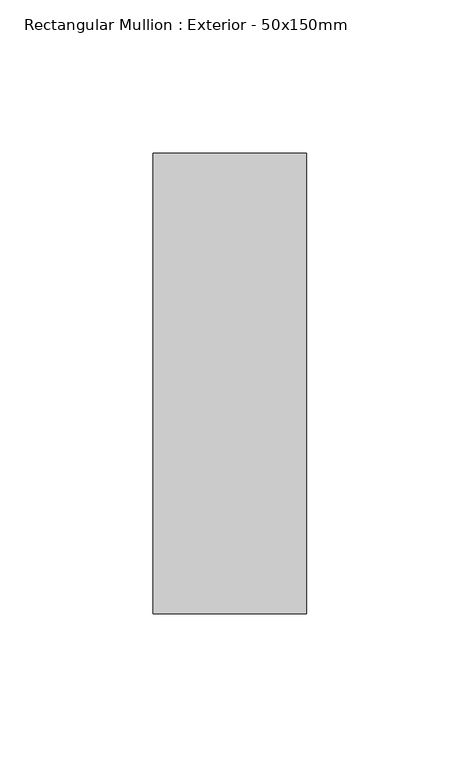
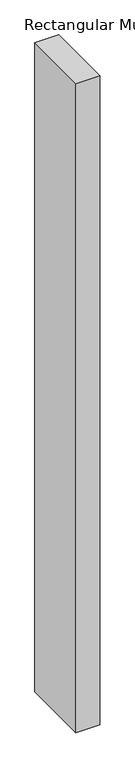
"""IFC4 building model written with IfcOpenShell, lengths in millimetres: member geometry, Rectangular Mullion : Exterior - 50x150mm."""

from ifc_helpers import new_model, si_unit, frame, origin, place, context, project, spatial, polyline, outline, extrude, source, transform, mapped, element, save


def rectangular_mullion_exterior_50x150mm_c96db089(model_context):
    return source(origin(), model_context, "Body", "SweptSolid", [
        extrude(outline(polyline([(0.0, 0.0), (0.0, -150.0), (-50.0, -150.0), (-50.0, 0.0), (0.0, 0.0)])), frame((0.0, 0.0, -1449.9999999), z_axis=(0.0, 0.0, 1.0), x_axis=(1.0, 0.0, 0.0)), (0.0, 0.0, 1.0), 1449.9999999),
    ])


if __name__ == "__main__":
    model = new_model("IFC4")
    model_context = context("Model", 3, world=origin())
    ifc_project = project(units=[si_unit("LENGTHUNIT", "METRE", prefix="MILLI")], contexts=[model_context])
    site = spatial("IfcSite", under=ifc_project)
    building = spatial("IfcBuilding", under=site)
    placement = place(None, origin())
    rectangular_mullion_exterior_50x150mm_shape = rectangular_mullion_exterior_50x150mm_c96db089(model_context)
    element("IfcMember", 1, ObjectType="Rectangular Mullion : Exterior - 50x150mm", at=placement, inside=building, context=model_context, shape_type="MappedRepresentation", body=[
        mapped(rectangular_mullion_exterior_50x150mm_shape, transform((0.0, 0.0, 0.0), x_axis=(1.0, 0.0, 0.0), y_axis=(0.0, 1.0, 0.0), z_axis=(0.0, 0.0, 1.0))),
    ])
    save(model, "model.ifc")

# Revit data of these elements
# Type "Rectangular Mullion : Exterior - 50x150mm"
#   built-in parameter 1007351 = -0.246063 (stored number, unit not read)
#   built-in parameter 1007304 = 0.492126 (stored number, unit not read)
#   built-in parameter 1007301 = 0.082021 (stored number, unit not read)
#   built-in parameter 1007300 = 0.082021 (stored number, unit not read)
# Element 1 (IfcMember, "Rectangular Mullion : Exterior - 50x150mm")
#   Materials on its faces: "Default Frame/Mullion (Interior/Exterior)"
# Materials
#   "Default Frame/Mullion (Interior/Exterior)": class "Generic", colour RGB 205 205 205, transparency 0, Description = "Udefineret karm/ramme materiale", Cost = 0
